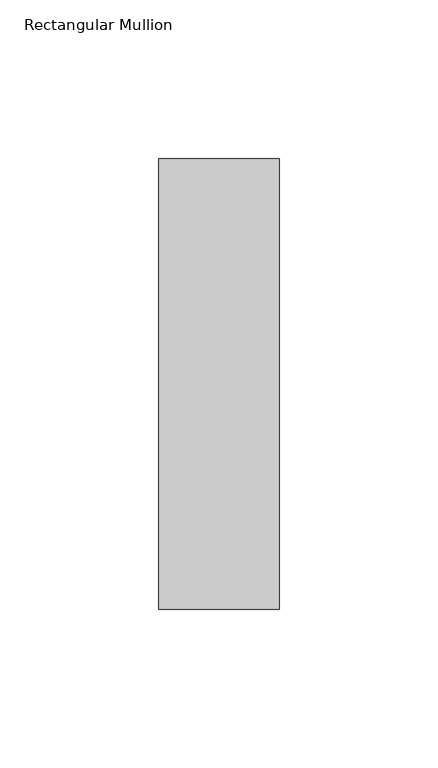
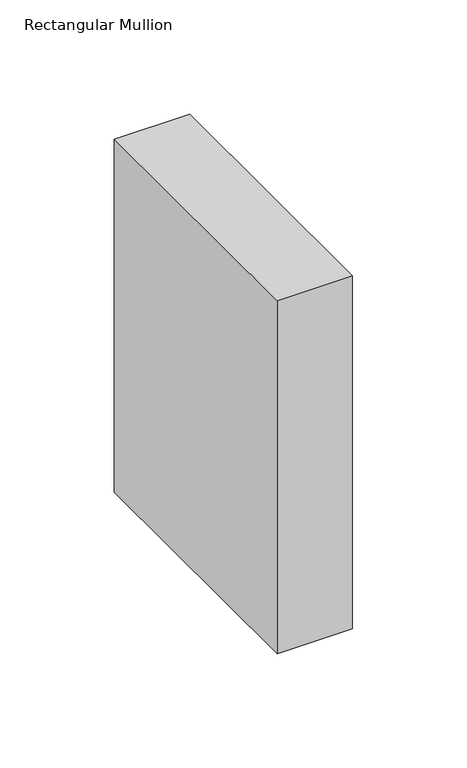
"""IFC4 building model written with IfcOpenShell, lengths in millimetres: member geometry, Rectangular Mullion : NLRS_21_CWM_hsb-regel 38x142_gen_rsf."""

from ifc_helpers import new_model, si_unit, frame, origin, place, context, project, spatial, polyline, outline, extrude, source, transform, mapped, element, save


def rectangular_mullion_03fbd13c(model_context):
    return source(origin(), model_context, "Body", "SweptSolid", [
        extrude(outline(polyline([(0.0, -71.0), (-38.0, -71.0), (-38.0, 71.0), (0.0, 71.0), (0.0, -71.0)])), frame((0.0, 0.0, -188.0000003), z_axis=(0.0, 0.0, 1.0), x_axis=(1.0, 0.0, 0.0)), (0.0, 0.0, 1.0), 188.0000003),
    ])


if __name__ == "__main__":
    model = new_model("IFC4")
    model_context = context("Model", 3, world=origin())
    ifc_project = project(units=[si_unit("LENGTHUNIT", "METRE", prefix="MILLI")], contexts=[model_context])
    site = spatial("IfcSite", under=ifc_project)
    building = spatial("IfcBuilding", under=site)
    placement = place(None, origin())
    rectangular_mullion_shape = rectangular_mullion_03fbd13c(model_context)
    element("IfcMember", 1, ObjectType="Rectangular Mullion : NLRS_21_CWM_hsb-regel 38x142_gen_rsf", at=placement, inside=building, context=model_context, shape_type="MappedRepresentation", body=[
        mapped(rectangular_mullion_shape, transform((0.0, 0.0, 0.0), x_axis=(1.0, 0.0, 0.0), y_axis=(0.0, 1.0, 0.0), z_axis=(0.0, 0.0, 1.0))),
    ])
    save(model, "model.ifc")

# Revit data of these elements
# Type "Rectangular Mullion : NLRS_21_CWM_hsb-regel 38x142_gen_rsf"
#   Export Type to IFC As = "IfcWall"
#   Type IfcGUID = "07M7mRoiH1CR8m_RSKIwpF"
#   Assembly Code = "21.10"
#   built-in parameter 1007322 = 0.465879 (stored number, unit not read)
#   built-in parameter 1007321 = 0.062336 (stored number, unit not read)
#   built-in parameter 1007320 = 0.062336 (stored number, unit not read)
# Element 1 (IfcMember, "Rectangular Mullion : NLRS_21_CWM_hsb-regel 38x142_gen_rsf")
#   Materials on its faces: "NLRS_i2_hout naaldhout vuren_gen_rsf"
# Materials
#   "NLRS_i2_hout naaldhout vuren_gen_rsf": class "I - Hout", colour RGB 234 199 147, transparency 0, Keynote = "i2", Manufacturer = "Revit Standards Foundation", URL = "www.revitstandards.org", Description = "hout vuren", Cost = 0
